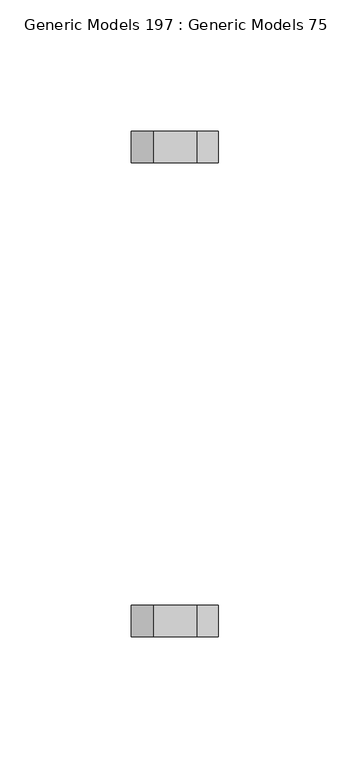
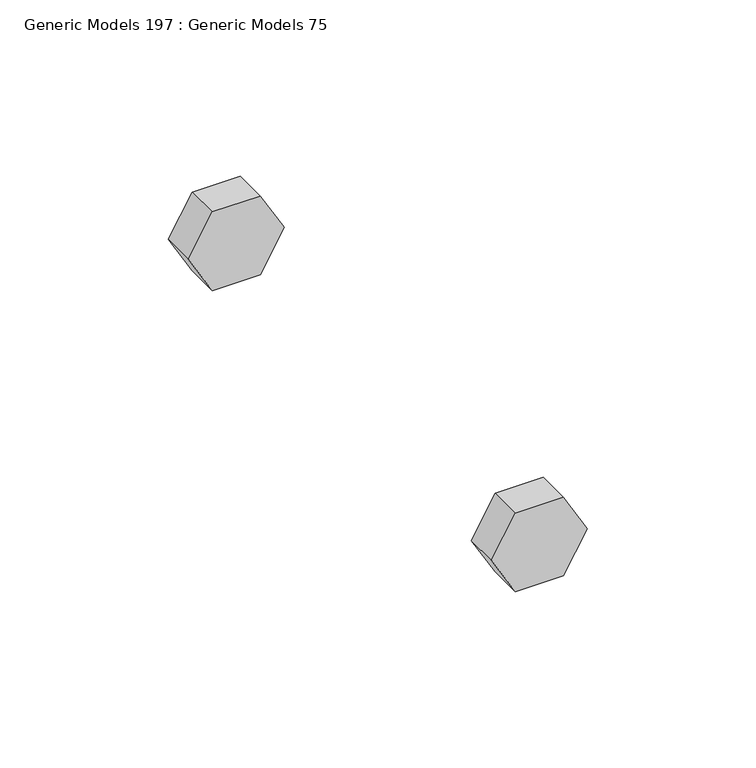
"""IFC4 building model written with IfcOpenShell, lengths in millimetres: proxy geometry, Generic Models 197 : Generic Models 75."""

from ifc_helpers import new_model, si_unit, frame, origin, place, context, project, spatial, polyline, outline, extrude, source, transform, mapped, element, save


def generic_models_197_generic_models_75_ac2514aa(model_context):
    return source(origin(), model_context, "Body", "SweptSolid", [
        extrude(outline(polyline([(271505.3625, 31978.2851858), (271505.3625, 31994.7829698), (271519.65, 32003.0318618), (271533.9375, 31994.7829698), (271533.9375, 31978.2851858), (271519.65, 31970.0362939), (271505.3625, 31978.2851858)])), frame((0.0, 30678.2969112, 0.0), z_axis=(0.0, 1.0, 0.0), x_axis=(0.0, 0.0, 1.0)), (0.0, 0.0, 1.0), 11.90625),
        extrude(outline(polyline([(271505.3625, 31978.2851858), (271505.3625, 31994.7829698), (271519.65, 32003.0318618), (271533.9375, 31994.7829698), (271533.9375, 31978.2851858), (271519.65, 31970.0362939), (271505.3625, 31978.2851858)])), frame((0.0, 30858.4781612, 0.0), z_axis=(0.0, 1.0, 0.0), x_axis=(0.0, 0.0, 1.0)), (0.0, 0.0, 1.0), 11.90625),
    ])


if __name__ == "__main__":
    model = new_model("IFC4")
    model_context = context("Model", 3, world=origin())
    ifc_project = project(units=[si_unit("LENGTHUNIT", "METRE", prefix="MILLI")], contexts=[model_context])
    site = spatial("IfcSite", under=ifc_project)
    building = spatial("IfcBuilding", under=site)
    placement = place(None, origin())
    generic_models_197_generic_models_75_shape = generic_models_197_generic_models_75_ac2514aa(model_context)
    element("IfcBuildingElementProxy", 1, Name="Generic Models 197 : Generic Models 75", ObjectType="Generic Models 197 : Generic Models 75", at=placement, inside=building, context=model_context, shape_type="MappedRepresentation", body=[
        mapped(generic_models_197_generic_models_75_shape, transform((0.0, 0.0, 0.0), x_axis=(1.0, 0.0, 0.0), y_axis=(0.0, 1.0, 0.0), z_axis=(0.0, 0.0, 1.0))),
    ])
    save(model, "model.ifc")

# Revit data of these elements
# Element 1 (IfcBuildingElementProxy, "Generic Models 197 : Generic Models 75")
#   Materials on its faces: "3/4\" GALV. THRU BOLTS"
# Materials
#   "3/4\" GALV. THRU BOLTS": class "Generic", colour RGB 105 69 171, transparency 0, Cost = 0
